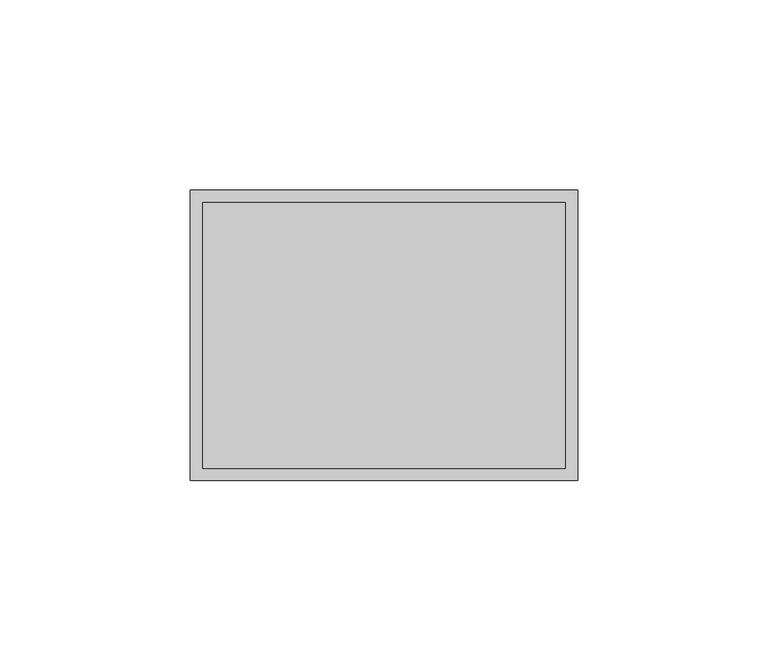
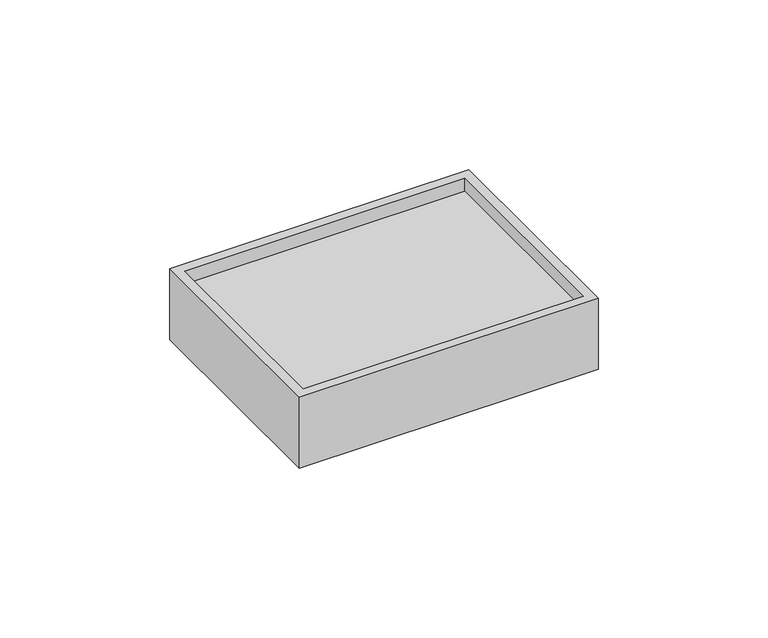
"""IFC4 building model written with IfcOpenShell, lengths in millimetres: proxy geometry, Soap Dish - NON-COLLECTUS : -."""

from ifc_helpers import new_model, si_unit, origin, place, context, project, spatial, faceted_brep, source, transform, mapped, element, save


def specialty_equipment_a8504747(model_context):
    return source(origin(), model_context, "Body", "Brep", [
        faceted_brep([(50.8, -76.2, 25.4), (-50.8, -76.2, 25.4), (-50.8, -76.2, 0.0), (50.8, -76.2, 0.0), (50.8, 0.0, 25.4), (50.8, 0.0, 0.0), (-50.8, 0.0, 0.0), (-50.8, 0.0, 25.4), (-47.625, -73.025, 25.4), (-47.625, -3.175, 25.4), (47.625, -3.175, 25.4), (47.625, -73.025, 25.4), (-47.625, -3.175, 20.6917529), (-47.625, -73.025, 20.6917529), (47.625, -73.025, 20.6917529), (47.625, -3.175, 20.6917529)], [[[0, 1, 2, 3]], [[4, 5, 6, 7]], [[1, 0, 4, 7], [8, 9, 10, 11]], [[2, 1, 7, 6]], [[3, 2, 6, 5]], [[0, 3, 5, 4]], [[12, 13, 14, 15]], [[13, 12, 9, 8]], [[14, 13, 8, 11]], [[15, 14, 11, 10]], [[12, 15, 10, 9]]]),
    ])


if __name__ == "__main__":
    model = new_model("IFC4")
    model_context = context("Model", 3, world=origin())
    ifc_project = project(units=[si_unit("LENGTHUNIT", "METRE", prefix="MILLI")], contexts=[model_context])
    site = spatial("IfcSite", under=ifc_project)
    building = spatial("IfcBuilding", under=site)
    placement = place(None, origin())
    specialty_equipment_shape = specialty_equipment_a8504747(model_context)
    element("IfcBuildingElementProxy", 1, Name="Soap Dish - NON-COLLECTUS : -", ObjectType="Soap Dish - NON-COLLECTUS : -", at=placement, inside=building, context=model_context, shape_type="MappedRepresentation", body=[
        mapped(specialty_equipment_shape, transform((0.0, 0.0, 0.0), x_axis=(1.0, 0.0, 0.0), y_axis=(0.0, 1.0, 0.0), z_axis=(0.0, 0.0, 1.0))),
    ])
    save(model, "model.ifc")

# Revit data of these elements
# Type "Soap Dish - NON-COLLECTUS : -"
#   External ID [instance default] = ""
#   Width = 101.6 mm
#   Height = 25.4 mm
#   Depth = 76.2 mm
#   Material = Light Grey
#   Default Elevation = 0
# Element 1 (IfcBuildingElementProxy, "Soap Dish - NON-COLLECTUS : -")
#   Materials on its faces: "Light Grey"
# Materials
#   "Light Grey": class "Generic", colour RGB 215 215 215, transparency 0, Cost = 0
